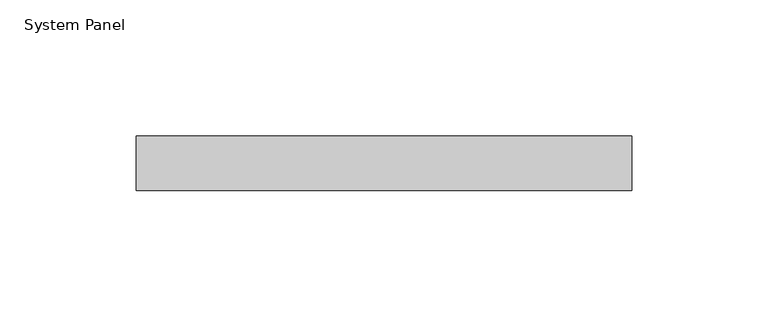
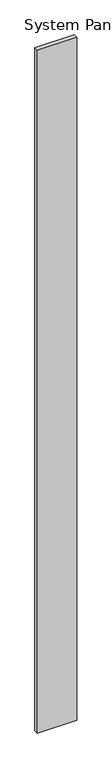
"""IFC4 building model written with IfcOpenShell, lengths in millimetres: plate geometry, System Panel : WWm-Glass-20mm-10mmOffset."""

from ifc_helpers import new_model, si_unit, origin, origin_with_axes, place, context, project, spatial, polyline, outline, extrude, source, transform, mapped, element, save


def system_panel_99f1046d(model_context):
    return source(origin(), model_context, "Body", "SweptSolid", [
        extrude(outline(polyline([(91.0, 0.0), (-91.0, 0.0), (-91.0, 20.0), (91.0, 20.0), (91.0, 0.0)])), origin_with_axes(), (0.0, 0.0, 1.0), 3350.0),
    ])


if __name__ == "__main__":
    model = new_model("IFC4")
    model_context = context("Model", 3, world=origin())
    ifc_project = project(units=[si_unit("LENGTHUNIT", "METRE", prefix="MILLI")], contexts=[model_context])
    site = spatial("IfcSite", under=ifc_project)
    building = spatial("IfcBuilding", under=site)
    placement = place(None, origin())
    system_panel_shape = system_panel_99f1046d(model_context)
    element("IfcPlate", 1, ObjectType="System Panel : WWm-Glass-20mm-10mmOffset", at=placement, inside=building, context=model_context, shape_type="MappedRepresentation", body=[
        mapped(system_panel_shape, transform((0.0, 0.0, 0.0), x_axis=(1.0, 0.0, 0.0), y_axis=(0.0, 1.0, 0.0), z_axis=(0.0, 0.0, 1.0))),
    ])
    save(model, "model.ifc")

# Revit data of these elements
# Type "System Panel : WWm-Glass-20mm-10mmOffset"
#   Finish = ""
# Element 1 (IfcPlate, "System Panel : WWm-Glass-20mm-10mmOffset")
#   Materials on its faces: "WW-EC-GL-Storefront"
# Materials
#   "WW-EC-GL-Storefront": class "Glass", colour RGB 236 240 239, transparency 0.85, Description = "Storefront Glass", Cost = 0
